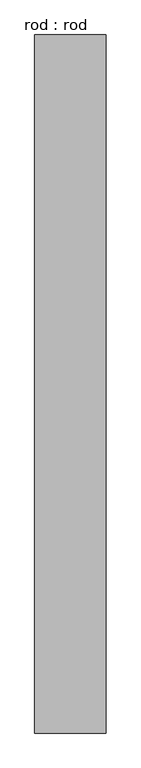
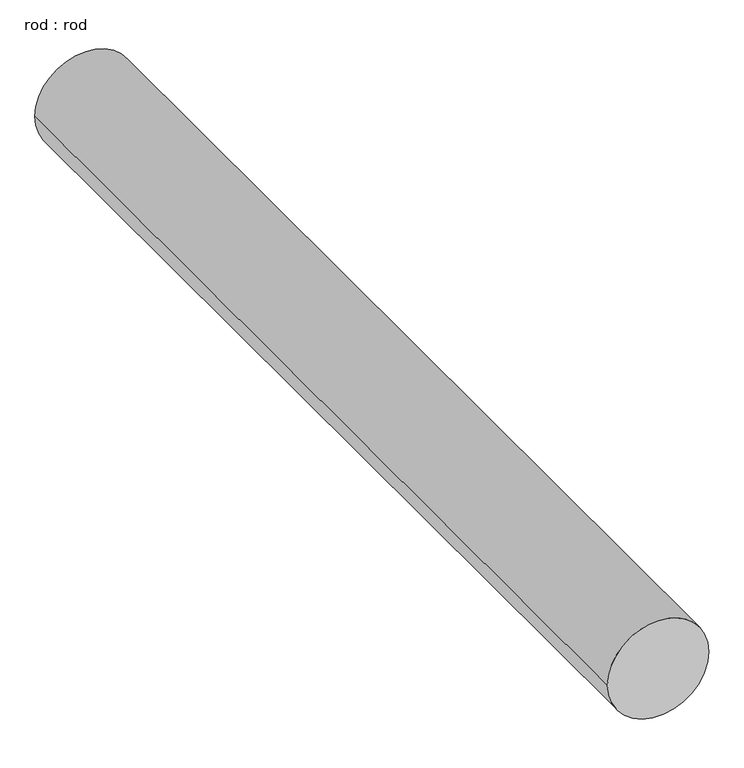
"""IFC4 building model written with IfcOpenShell, lengths in millimetres: proxy geometry, rod : rod."""

from ifc_helpers import new_model, si_unit, point, frame, frame_2d, origin, place, context, project, spatial, circle_curve, trimmed, segment, composite_curve, outline, extrude, source, transform, mapped, element, save


def rod_rod_523c131a(model_context):
    return source(origin(), model_context, "Body", "SweptSolid", [
        extrude(outline(composite_curve([segment(trimmed(circle_curve(frame_2d((0.0108462, 0.0)), 200.0), [point((0.0108462, 200.0))], [point((0.0108462, -200.0))], False, "CARTESIAN"), True, "CONTINUOUS"), segment(trimmed(circle_curve(frame_2d((0.0108462, 0.0)), 200.0), [point((0.0108462, -200.0))], [point((0.0108462, 200.0))], False, "CARTESIAN"), True, "CONTINUOUS")], self_intersect=False)), frame((0.0, 2134.373119, 0.0), z_axis=(0.0, 1.0, 0.0), x_axis=(0.0, 0.0, 1.0)), (0.0, 0.0, 1.0), 3916.7109927),
    ])


if __name__ == "__main__":
    model = new_model("IFC4")
    model_context = context("Model", 3, world=origin())
    ifc_project = project(units=[si_unit("LENGTHUNIT", "METRE", prefix="MILLI")], contexts=[model_context])
    site = spatial("IfcSite", under=ifc_project)
    building = spatial("IfcBuilding", under=site)
    placement = place(None, origin())
    rod_rod_shape = rod_rod_523c131a(model_context)
    element("IfcBuildingElementProxy", 1, Name="rod : rod", ObjectType="rod : rod", at=placement, inside=building, context=model_context, shape_type="MappedRepresentation", body=[
        mapped(rod_rod_shape, transform((0.0, 0.0, 0.0), x_axis=(1.0, 0.0, 0.0), y_axis=(0.0, 1.0, 0.0), z_axis=(0.0, 0.0, 1.0))),
    ])
    save(model, "model.ifc")

# Revit data of these elements
# Type "rod : rod"
#   Default Elevation = 0
